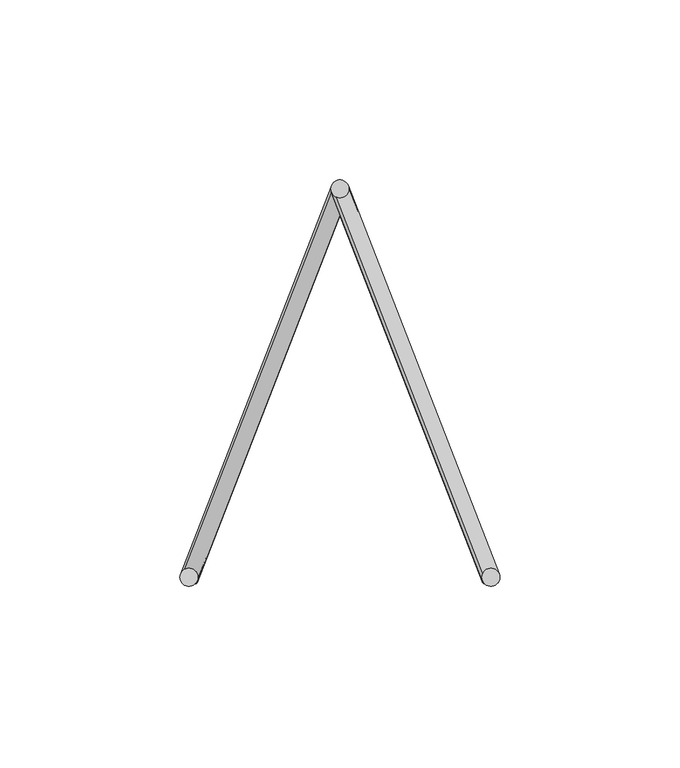
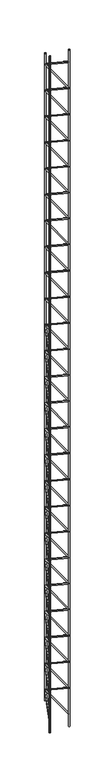
"""IFC4 building model written with IfcOpenShell, lengths in millimetres: proxy geometry, Pre-fab. (Vigota 2 - Pano 4)."""

from ifc_helpers import new_model, si_unit, point, frame, frame_2d, origin, origin_with_axes, origin_2d, place, context, project, spatial, circle_curve, trimmed, segment, composite_curve, outline, extrude, source, transform, mapped, element, save


def structural_framing_4307f6da(model_context):
    return source(origin(), model_context, "Body", "SweptSolid", [
        extrude(outline(composite_curve([segment(trimmed(circle_curve(origin_2d(), 2.5), [point((2.5, 0.0))], [point((-2.5, 0.0))], False, "CARTESIAN"), True, "CONTINUOUS"), segment(trimmed(circle_curve(origin_2d(), 2.5), [point((-2.5, 0.0))], [point((2.5, 0.0))], False, "CARTESIAN"), True, "CONTINUOUS")], self_intersect=False)), origin_with_axes(), (0.0, 0.0, 1.0), 3114.0),
        extrude(outline(composite_curve([segment(trimmed(circle_curve(frame_2d((-42.0, 108.0)), 2.5), [point((-39.5, 108.0))], [point((-44.5, 108.0))], False, "CARTESIAN"), True, "CONTINUOUS"), segment(trimmed(circle_curve(frame_2d((-42.0, 108.0)), 2.5), [point((-44.5, 108.0))], [point((-39.5, 108.0))], False, "CARTESIAN"), True, "CONTINUOUS")], self_intersect=False)), frame((0.0, 0.0, 67.0), z_axis=(0.0, 0.0, 1.0), x_axis=(1.0, 0.0, 0.0)), (0.0, 0.0, 1.0), 2980.0),
        extrude(outline(composite_curve([segment(trimmed(circle_curve(origin_2d(), 2.5), [point((2.5, 0.0))], [point((-2.5, 0.0))], False, "CARTESIAN"), True, "CONTINUOUS"), segment(trimmed(circle_curve(origin_2d(), 2.5), [point((-2.5, 0.0))], [point((2.5, 0.0))], False, "CARTESIAN"), True, "CONTINUOUS")], self_intersect=False)), frame((0.0, 0.0, 57.0), z_axis=(-0.3218603428886276, 0.8276408817707567, 0.4598004898837537), x_axis=(0.8192319205108605, -3.936835275445103e-11, 0.5734623443750141)), (0.0, 0.0, 1.0), 130.491379),
        extrude(outline(composite_curve([segment(trimmed(circle_curve(origin_2d(), 2.5), [point((2.5, 0.0))], [point((-2.5, 0.0))], False, "CARTESIAN"), True, "CONTINUOUS"), segment(trimmed(circle_curve(origin_2d(), 2.5), [point((-2.5, 0.0))], [point((2.5, 0.0))], False, "CARTESIAN"), True, "CONTINUOUS")], self_intersect=False)), frame((-42.0, 108.0, 117.0), z_axis=(0.3218603428886276, -0.8276408817707567, 0.4598004898837537), x_axis=(0.8192319205108605, -3.936835275445103e-11, -0.5734623443750141)), (0.0, 0.0, 1.0), 130.491379),
        extrude(outline(composite_curve([segment(trimmed(circle_curve(origin_2d(), 2.5), [point((2.5, 0.0))], [point((-2.5, 0.0))], False, "CARTESIAN"), True, "CONTINUOUS"), segment(trimmed(circle_curve(origin_2d(), 2.5), [point((-2.5, 0.0))], [point((2.5, 0.0))], False, "CARTESIAN"), True, "CONTINUOUS")], self_intersect=False)), frame((0.0, 0.0, 177.0), z_axis=(-0.3218603428886276, 0.8276408817707567, 0.4598004898837537), x_axis=(0.8192319205108605, -3.936835275445103e-11, 0.5734623443750141)), (0.0, 0.0, 1.0), 130.491379),
        extrude(outline(composite_curve([segment(trimmed(circle_curve(origin_2d(), 2.5), [point((2.5, 0.0))], [point((-2.5, 0.0))], False, "CARTESIAN"), True, "CONTINUOUS"), segment(trimmed(circle_curve(origin_2d(), 2.5), [point((-2.5, 0.0))], [point((2.5, 0.0))], False, "CARTESIAN"), True, "CONTINUOUS")], self_intersect=False)), frame((-42.0, 108.0, 237.0), z_axis=(0.3218603428886276, -0.8276408817707567, 0.4598004898837537), x_axis=(0.8192319205108605, -3.936835275445103e-11, -0.5734623443750141)), (0.0, 0.0, 1.0), 130.491379),
        extrude(outline(composite_curve([segment(trimmed(circle_curve(origin_2d(), 2.5), [point((2.5, 0.0))], [point((-2.5, 0.0))], False, "CARTESIAN"), True, "CONTINUOUS"), segment(trimmed(circle_curve(origin_2d(), 2.5), [point((-2.5, 0.0))], [point((2.5, 0.0))], False, "CARTESIAN"), True, "CONTINUOUS")], self_intersect=False)), frame((0.0, 0.0, 297.0), z_axis=(-0.3218603428886276, 0.8276408817707567, 0.4598004898837537), x_axis=(0.8192319205108605, -3.936835275445103e-11, 0.5734623443750141)), (0.0, 0.0, 1.0), 130.491379),
        extrude(outline(composite_curve([segment(trimmed(circle_curve(origin_2d(), 2.5), [point((2.5, 0.0))], [point((-2.5, 0.0))], False, "CARTESIAN"), True, "CONTINUOUS"), segment(trimmed(circle_curve(origin_2d(), 2.5), [point((-2.5, 0.0))], [point((2.5, 0.0))], False, "CARTESIAN"), True, "CONTINUOUS")], self_intersect=False)), frame((-42.0, 108.0, 357.0), z_axis=(0.3218603428886276, -0.8276408817707567, 0.4598004898837537), x_axis=(0.8192319205108605, -3.936835275445103e-11, -0.5734623443750141)), (0.0, 0.0, 1.0), 130.491379),
        extrude(outline(composite_curve([segment(trimmed(circle_curve(origin_2d(), 2.5), [point((2.5, 0.0))], [point((-2.5, 0.0))], False, "CARTESIAN"), True, "CONTINUOUS"), segment(trimmed(circle_curve(origin_2d(), 2.5), [point((-2.5, 0.0))], [point((2.5, 0.0))], False, "CARTESIAN"), True, "CONTINUOUS")], self_intersect=False)), frame((0.0, 0.0, 417.0), z_axis=(-0.3218603428886276, 0.8276408817707567, 0.4598004898837537), x_axis=(0.8192319205108605, -3.936835275445103e-11, 0.5734623443750141)), (0.0, 0.0, 1.0), 130.491379),
        extrude(outline(composite_curve([segment(trimmed(circle_curve(origin_2d(), 2.5), [point((2.5, 0.0))], [point((-2.5, 0.0))], False, "CARTESIAN"), True, "CONTINUOUS"), segment(trimmed(circle_curve(origin_2d(), 2.5), [point((-2.5, 0.0))], [point((2.5, 0.0))], False, "CARTESIAN"), True, "CONTINUOUS")], self_intersect=False)), frame((-42.0, 108.0, 477.0), z_axis=(0.3218603428886276, -0.8276408817707567, 0.4598004898837537), x_axis=(0.8192319205108605, -3.936835275445103e-11, -0.5734623443750141)), (0.0, 0.0, 1.0), 130.491379),
        extrude(outline(composite_curve([segment(trimmed(circle_curve(origin_2d(), 2.5), [point((2.5, 0.0))], [point((-2.5, 0.0))], False, "CARTESIAN"), True, "CONTINUOUS"), segment(trimmed(circle_curve(origin_2d(), 2.5), [point((-2.5, 0.0))], [point((2.5, 0.0))], False, "CARTESIAN"), True, "CONTINUOUS")], self_intersect=False)), frame((0.0, 0.0, 537.0), z_axis=(-0.3218603428886276, 0.8276408817707567, 0.4598004898837537), x_axis=(0.8192319205108605, -3.936835275445103e-11, 0.5734623443750141)), (0.0, 0.0, 1.0), 130.491379),
        extrude(outline(composite_curve([segment(trimmed(circle_curve(origin_2d(), 2.5), [point((2.5, 0.0))], [point((-2.5, 0.0))], False, "CARTESIAN"), True, "CONTINUOUS"), segment(trimmed(circle_curve(origin_2d(), 2.5), [point((-2.5, 0.0))], [point((2.5, 0.0))], False, "CARTESIAN"), True, "CONTINUOUS")], self_intersect=False)), frame((-42.0, 108.0, 597.0), z_axis=(0.3218603428886276, -0.8276408817707567, 0.4598004898837537), x_axis=(0.8192319205108605, -3.936835275445103e-11, -0.5734623443750141)), (0.0, 0.0, 1.0), 130.491379),
        extrude(outline(composite_curve([segment(trimmed(circle_curve(origin_2d(), 2.5), [point((2.5, 0.0))], [point((-2.5, 0.0))], False, "CARTESIAN"), True, "CONTINUOUS"), segment(trimmed(circle_curve(origin_2d(), 2.5), [point((-2.5, 0.0))], [point((2.5, 0.0))], False, "CARTESIAN"), True, "CONTINUOUS")], self_intersect=False)), frame((0.0, 0.0, 657.0), z_axis=(-0.3218603428886276, 0.8276408817707567, 0.4598004898837537), x_axis=(0.8192319205108605, -3.936835275445103e-11, 0.5734623443750141)), (0.0, 0.0, 1.0), 130.491379),
        extrude(outline(composite_curve([segment(trimmed(circle_curve(origin_2d(), 2.5), [point((2.5, 0.0))], [point((-2.5, 0.0))], False, "CARTESIAN"), True, "CONTINUOUS"), segment(trimmed(circle_curve(origin_2d(), 2.5), [point((-2.5, 0.0))], [point((2.5, 0.0))], False, "CARTESIAN"), True, "CONTINUOUS")], self_intersect=False)), frame((-42.0, 108.0, 717.0), z_axis=(0.3218603428886276, -0.8276408817707567, 0.4598004898837537), x_axis=(0.8192319205108605, -3.936835275445103e-11, -0.5734623443750141)), (0.0, 0.0, 1.0), 130.491379),
        extrude(outline(composite_curve([segment(trimmed(circle_curve(origin_2d(), 2.5), [point((2.5, 0.0))], [point((-2.5, 0.0))], False, "CARTESIAN"), True, "CONTINUOUS"), segment(trimmed(circle_curve(origin_2d(), 2.5), [point((-2.5, 0.0))], [point((2.5, 0.0))], False, "CARTESIAN"), True, "CONTINUOUS")], self_intersect=False)), frame((0.0, 0.0, 777.0), z_axis=(-0.3218603428886276, 0.8276408817707567, 0.4598004898837537), x_axis=(0.8192319205108605, -3.936835275445103e-11, 0.5734623443750141)), (0.0, 0.0, 1.0), 130.491379),
        extrude(outline(composite_curve([segment(trimmed(circle_curve(origin_2d(), 2.5), [point((2.5, 0.0))], [point((-2.5, 0.0))], False, "CARTESIAN"), True, "CONTINUOUS"), segment(trimmed(circle_curve(origin_2d(), 2.5), [point((-2.5, 0.0))], [point((2.5, 0.0))], False, "CARTESIAN"), True, "CONTINUOUS")], self_intersect=False)), frame((-42.0, 108.0, 837.0), z_axis=(0.3218603428886276, -0.8276408817707567, 0.4598004898837537), x_axis=(0.8192319205108605, -3.936835275445103e-11, -0.5734623443750141)), (0.0, 0.0, 1.0), 130.491379),
        extrude(outline(composite_curve([segment(trimmed(circle_curve(origin_2d(), 2.5), [point((2.5, 0.0))], [point((-2.5, 0.0))], False, "CARTESIAN"), True, "CONTINUOUS"), segment(trimmed(circle_curve(origin_2d(), 2.5), [point((-2.5, 0.0))], [point((2.5, 0.0))], False, "CARTESIAN"), True, "CONTINUOUS")], self_intersect=False)), frame((0.0, 0.0, 897.0), z_axis=(-0.3218603428886276, 0.8276408817707567, 0.4598004898837537), x_axis=(0.8192319205108605, -3.936835275445103e-11, 0.5734623443750141)), (0.0, 0.0, 1.0), 130.491379),
        extrude(outline(composite_curve([segment(trimmed(circle_curve(origin_2d(), 2.5), [point((2.5, 0.0))], [point((-2.5, 0.0))], False, "CARTESIAN"), True, "CONTINUOUS"), segment(trimmed(circle_curve(origin_2d(), 2.5), [point((-2.5, 0.0))], [point((2.5, 0.0))], False, "CARTESIAN"), True, "CONTINUOUS")], self_intersect=False)), frame((-42.0, 108.0, 957.0), z_axis=(0.3218603428886276, -0.8276408817707567, 0.4598004898837537), x_axis=(0.8192319205108605, -3.936835275445103e-11, -0.5734623443750141)), (0.0, 0.0, 1.0), 130.491379),
        extrude(outline(composite_curve([segment(trimmed(circle_curve(origin_2d(), 2.5), [point((2.5, 0.0))], [point((-2.5, 0.0))], False, "CARTESIAN"), True, "CONTINUOUS"), segment(trimmed(circle_curve(origin_2d(), 2.5), [point((-2.5, 0.0))], [point((2.5, 0.0))], False, "CARTESIAN"), True, "CONTINUOUS")], self_intersect=False)), frame((0.0, 0.0, 1017.0), z_axis=(-0.3218603428886276, 0.8276408817707567, 0.4598004898837537), x_axis=(0.8192319205108605, -3.936835275445103e-11, 0.5734623443750141)), (0.0, 0.0, 1.0), 130.491379),
        extrude(outline(composite_curve([segment(trimmed(circle_curve(origin_2d(), 2.5), [point((2.5, 0.0))], [point((-2.5, 0.0))], False, "CARTESIAN"), True, "CONTINUOUS"), segment(trimmed(circle_curve(origin_2d(), 2.5), [point((-2.5, 0.0))], [point((2.5, 0.0))], False, "CARTESIAN"), True, "CONTINUOUS")], self_intersect=False)), frame((-42.0, 108.0, 1077.0), z_axis=(0.3218603428886276, -0.8276408817707567, 0.4598004898837537), x_axis=(0.8192319205108605, -3.936835275445103e-11, -0.5734623443750141)), (0.0, 0.0, 1.0), 130.491379),
        extrude(outline(composite_curve([segment(trimmed(circle_curve(origin_2d(), 2.5), [point((2.5, 0.0))], [point((-2.5, 0.0))], False, "CARTESIAN"), True, "CONTINUOUS"), segment(trimmed(circle_curve(origin_2d(), 2.5), [point((-2.5, 0.0))], [point((2.5, 0.0))], False, "CARTESIAN"), True, "CONTINUOUS")], self_intersect=False)), frame((0.0, 0.0, 1137.0), z_axis=(-0.3218603428886276, 0.8276408817707567, 0.4598004898837537), x_axis=(0.8192319205108605, -3.936835275445103e-11, 0.5734623443750141)), (0.0, 0.0, 1.0), 130.491379),
        extrude(outline(composite_curve([segment(trimmed(circle_curve(origin_2d(), 2.5), [point((2.5, 0.0))], [point((-2.5, 0.0))], False, "CARTESIAN"), True, "CONTINUOUS"), segment(trimmed(circle_curve(origin_2d(), 2.5), [point((-2.5, 0.0))], [point((2.5, 0.0))], False, "CARTESIAN"), True, "CONTINUOUS")], self_intersect=False)), frame((-42.0, 108.0, 1197.0), z_axis=(0.3218603428886276, -0.8276408817707567, 0.4598004898837537), x_axis=(0.8192319205108605, -3.936835275445103e-11, -0.5734623443750141)), (0.0, 0.0, 1.0), 130.491379),
        extrude(outline(composite_curve([segment(trimmed(circle_curve(origin_2d(), 2.5), [point((2.5, 0.0))], [point((-2.5, 0.0))], False, "CARTESIAN"), True, "CONTINUOUS"), segment(trimmed(circle_curve(origin_2d(), 2.5), [point((-2.5, 0.0))], [point((2.5, 0.0))], False, "CARTESIAN"), True, "CONTINUOUS")], self_intersect=False)), frame((0.0, 0.0, 1257.0), z_axis=(-0.3218603428886276, 0.8276408817707567, 0.4598004898837537), x_axis=(0.8192319205108605, -3.936835275445103e-11, 0.5734623443750141)), (0.0, 0.0, 1.0), 130.491379),
        extrude(outline(composite_curve([segment(trimmed(circle_curve(origin_2d(), 2.5), [point((2.5, 0.0))], [point((-2.5, 0.0))], False, "CARTESIAN"), True, "CONTINUOUS"), segment(trimmed(circle_curve(origin_2d(), 2.5), [point((-2.5, 0.0))], [point((2.5, 0.0))], False, "CARTESIAN"), True, "CONTINUOUS")], self_intersect=False)), frame((-42.0, 108.0, 1317.0), z_axis=(0.3218603428886276, -0.8276408817707567, 0.4598004898837537), x_axis=(0.8192319205108605, -3.936835275445103e-11, -0.5734623443750141)), (0.0, 0.0, 1.0), 130.491379),
        extrude(outline(composite_curve([segment(trimmed(circle_curve(origin_2d(), 2.5), [point((2.5, 0.0))], [point((-2.5, 0.0))], False, "CARTESIAN"), True, "CONTINUOUS"), segment(trimmed(circle_curve(origin_2d(), 2.5), [point((-2.5, 0.0))], [point((2.5, 0.0))], False, "CARTESIAN"), True, "CONTINUOUS")], self_intersect=False)), frame((0.0, 0.0, 1377.0), z_axis=(-0.3218603428886276, 0.8276408817707567, 0.4598004898837537), x_axis=(0.8192319205108605, -3.936835275445103e-11, 0.5734623443750141)), (0.0, 0.0, 1.0), 130.491379),
        extrude(outline(composite_curve([segment(trimmed(circle_curve(origin_2d(), 2.5), [point((2.5, 0.0))], [point((-2.5, 0.0))], False, "CARTESIAN"), True, "CONTINUOUS"), segment(trimmed(circle_curve(origin_2d(), 2.5), [point((-2.5, 0.0))], [point((2.5, 0.0))], False, "CARTESIAN"), True, "CONTINUOUS")], self_intersect=False)), frame((-42.0, 108.0, 1437.0), z_axis=(0.3218603428886276, -0.8276408817707567, 0.4598004898837537), x_axis=(0.8192319205108605, -3.936835275445103e-11, -0.5734623443750141)), (0.0, 0.0, 1.0), 130.491379),
        extrude(outline(composite_curve([segment(trimmed(circle_curve(origin_2d(), 2.5), [point((2.5, 0.0))], [point((-2.5, 0.0))], False, "CARTESIAN"), True, "CONTINUOUS"), segment(trimmed(circle_curve(origin_2d(), 2.5), [point((-2.5, 0.0))], [point((2.5, 0.0))], False, "CARTESIAN"), True, "CONTINUOUS")], self_intersect=False)), frame((0.0, 0.0, 1497.0), z_axis=(-0.3218603428886276, 0.8276408817707567, 0.4598004898837537), x_axis=(0.8192319205108605, -3.936835275445103e-11, 0.5734623443750141)), (0.0, 0.0, 1.0), 130.491379),
        extrude(outline(composite_curve([segment(trimmed(circle_curve(origin_2d(), 2.5), [point((2.5, 0.0))], [point((-2.5, 0.0))], False, "CARTESIAN"), True, "CONTINUOUS"), segment(trimmed(circle_curve(origin_2d(), 2.5), [point((-2.5, 0.0))], [point((2.5, 0.0))], False, "CARTESIAN"), True, "CONTINUOUS")], self_intersect=False)), frame((-42.0, 108.0, 1557.0), z_axis=(0.3218603428886276, -0.8276408817707567, 0.4598004898837537), x_axis=(0.8192319205108605, -3.936835275445103e-11, -0.5734623443750141)), (0.0, 0.0, 1.0), 130.491379),
        extrude(outline(composite_curve([segment(trimmed(circle_curve(origin_2d(), 2.5), [point((2.5, 0.0))], [point((-2.5, 0.0))], False, "CARTESIAN"), True, "CONTINUOUS"), segment(trimmed(circle_curve(origin_2d(), 2.5), [point((-2.5, 0.0))], [point((2.5, 0.0))], False, "CARTESIAN"), True, "CONTINUOUS")], self_intersect=False)), frame((0.0, 0.0, 1617.0), z_axis=(-0.3218603428886276, 0.8276408817707567, 0.4598004898837537), x_axis=(0.8192319205108605, -3.936835275445103e-11, 0.5734623443750141)), (0.0, 0.0, 1.0), 130.491379),
        extrude(outline(composite_curve([segment(trimmed(circle_curve(origin_2d(), 2.5), [point((2.5, 0.0))], [point((-2.5, 0.0))], False, "CARTESIAN"), True, "CONTINUOUS"), segment(trimmed(circle_curve(origin_2d(), 2.5), [point((-2.5, 0.0))], [point((2.5, 0.0))], False, "CARTESIAN"), True, "CONTINUOUS")], self_intersect=False)), frame((-42.0, 108.0, 1677.0), z_axis=(0.3218603428886276, -0.8276408817707567, 0.4598004898837537), x_axis=(0.8192319205108605, -3.936835275445103e-11, -0.5734623443750141)), (0.0, 0.0, 1.0), 130.491379),
        extrude(outline(composite_curve([segment(trimmed(circle_curve(origin_2d(), 2.5), [point((2.5, 0.0))], [point((-2.5, 0.0))], False, "CARTESIAN"), True, "CONTINUOUS"), segment(trimmed(circle_curve(origin_2d(), 2.5), [point((-2.5, 0.0))], [point((2.5, 0.0))], False, "CARTESIAN"), True, "CONTINUOUS")], self_intersect=False)), frame((0.0, 0.0, 1737.0), z_axis=(-0.3218603428886276, 0.8276408817707567, 0.4598004898837537), x_axis=(0.8192319205108605, -3.936835275445103e-11, 0.5734623443750141)), (0.0, 0.0, 1.0), 130.491379),
        extrude(outline(composite_curve([segment(trimmed(circle_curve(origin_2d(), 2.5), [point((2.5, 0.0))], [point((-2.5, 0.0))], False, "CARTESIAN"), True, "CONTINUOUS"), segment(trimmed(circle_curve(origin_2d(), 2.5), [point((-2.5, 0.0))], [point((2.5, 0.0))], False, "CARTESIAN"), True, "CONTINUOUS")], self_intersect=False)), frame((-42.0, 108.0, 1797.0), z_axis=(0.3218603428886276, -0.8276408817707567, 0.4598004898837537), x_axis=(0.8192319205108605, -3.936835275445103e-11, -0.5734623443750141)), (0.0, 0.0, 1.0), 130.491379),
        extrude(outline(composite_curve([segment(trimmed(circle_curve(origin_2d(), 2.5), [point((2.5, 0.0))], [point((-2.5, 0.0))], False, "CARTESIAN"), True, "CONTINUOUS"), segment(trimmed(circle_curve(origin_2d(), 2.5), [point((-2.5, 0.0))], [point((2.5, 0.0))], False, "CARTESIAN"), True, "CONTINUOUS")], self_intersect=False)), frame((0.0, 0.0, 1857.0), z_axis=(-0.3218603428886276, 0.8276408817707567, 0.4598004898837537), x_axis=(0.8192319205108605, -3.936835275445103e-11, 0.5734623443750141)), (0.0, 0.0, 1.0), 130.491379),
        extrude(outline(composite_curve([segment(trimmed(circle_curve(origin_2d(), 2.5), [point((2.5, 0.0))], [point((-2.5, 0.0))], False, "CARTESIAN"), True, "CONTINUOUS"), segment(trimmed(circle_curve(origin_2d(), 2.5), [point((-2.5, 0.0))], [point((2.5, 0.0))], False, "CARTESIAN"), True, "CONTINUOUS")], self_intersect=False)), frame((-42.0, 108.0, 1917.0), z_axis=(0.3218603428886276, -0.8276408817707567, 0.4598004898837537), x_axis=(0.8192319205108605, -3.936835275445103e-11, -0.5734623443750141)), (0.0, 0.0, 1.0), 130.491379),
        extrude(outline(composite_curve([segment(trimmed(circle_curve(origin_2d(), 2.5), [point((2.5, 0.0))], [point((-2.5, 0.0))], False, "CARTESIAN"), True, "CONTINUOUS"), segment(trimmed(circle_curve(origin_2d(), 2.5), [point((-2.5, 0.0))], [point((2.5, 0.0))], False, "CARTESIAN"), True, "CONTINUOUS")], self_intersect=False)), frame((0.0, 0.0, 1977.0), z_axis=(-0.3218603428886276, 0.8276408817707567, 0.4598004898837537), x_axis=(0.8192319205108605, -3.936835275445103e-11, 0.5734623443750141)), (0.0, 0.0, 1.0), 130.491379),
        extrude(outline(composite_curve([segment(trimmed(circle_curve(origin_2d(), 2.5), [point((2.5, 0.0))], [point((-2.5, 0.0))], False, "CARTESIAN"), True, "CONTINUOUS"), segment(trimmed(circle_curve(origin_2d(), 2.5), [point((-2.5, 0.0))], [point((2.5, 0.0))], False, "CARTESIAN"), True, "CONTINUOUS")], self_intersect=False)), frame((-42.0, 108.0, 2037.0), z_axis=(0.3218603428886276, -0.8276408817707567, 0.4598004898837537), x_axis=(0.8192319205108605, -3.936835275445103e-11, -0.5734623443750141)), (0.0, 0.0, 1.0), 130.491379),
        extrude(outline(composite_curve([segment(trimmed(circle_curve(origin_2d(), 2.5), [point((2.5, 0.0))], [point((-2.5, 0.0))], False, "CARTESIAN"), True, "CONTINUOUS"), segment(trimmed(circle_curve(origin_2d(), 2.5), [point((-2.5, 0.0))], [point((2.5, 0.0))], False, "CARTESIAN"), True, "CONTINUOUS")], self_intersect=False)), frame((0.0, 0.0, 2097.0), z_axis=(-0.3218603428886276, 0.8276408817707567, 0.4598004898837537), x_axis=(0.8192319205108605, -3.936835275445103e-11, 0.5734623443750141)), (0.0, 0.0, 1.0), 130.491379),
        extrude(outline(composite_curve([segment(trimmed(circle_curve(origin_2d(), 2.5), [point((2.5, 0.0))], [point((-2.5, 0.0))], False, "CARTESIAN"), True, "CONTINUOUS"), segment(trimmed(circle_curve(origin_2d(), 2.5), [point((-2.5, 0.0))], [point((2.5, 0.0))], False, "CARTESIAN"), True, "CONTINUOUS")], self_intersect=False)), frame((-42.0, 108.0, 2157.0), z_axis=(0.3218603428886276, -0.8276408817707567, 0.4598004898837537), x_axis=(0.8192319205108605, -3.936835275445103e-11, -0.5734623443750141)), (0.0, 0.0, 1.0), 130.491379),
        extrude(outline(composite_curve([segment(trimmed(circle_curve(origin_2d(), 2.5), [point((2.5, 0.0))], [point((-2.5, 0.0))], False, "CARTESIAN"), True, "CONTINUOUS"), segment(trimmed(circle_curve(origin_2d(), 2.5), [point((-2.5, 0.0))], [point((2.5, 0.0))], False, "CARTESIAN"), True, "CONTINUOUS")], self_intersect=False)), frame((0.0, 0.0, 2217.0), z_axis=(-0.3218603428886276, 0.8276408817707567, 0.4598004898837537), x_axis=(0.8192319205108605, -3.936835275445103e-11, 0.5734623443750141)), (0.0, 0.0, 1.0), 130.491379),
        extrude(outline(composite_curve([segment(trimmed(circle_curve(origin_2d(), 2.5), [point((2.5, 0.0))], [point((-2.5, 0.0))], False, "CARTESIAN"), True, "CONTINUOUS"), segment(trimmed(circle_curve(origin_2d(), 2.5), [point((-2.5, 0.0))], [point((2.5, 0.0))], False, "CARTESIAN"), True, "CONTINUOUS")], self_intersect=False)), frame((-42.0, 108.0, 2277.0), z_axis=(0.3218603428886276, -0.8276408817707567, 0.4598004898837537), x_axis=(0.8192319205108605, -3.936835275445103e-11, -0.5734623443750141)), (0.0, 0.0, 1.0), 130.491379),
        extrude(outline(composite_curve([segment(trimmed(circle_curve(origin_2d(), 2.5), [point((2.5, 0.0))], [point((-2.5, 0.0))], False, "CARTESIAN"), True, "CONTINUOUS"), segment(trimmed(circle_curve(origin_2d(), 2.5), [point((-2.5, 0.0))], [point((2.5, 0.0))], False, "CARTESIAN"), True, "CONTINUOUS")], self_intersect=False)), frame((0.0, 0.0, 2337.0), z_axis=(-0.3218603428886276, 0.8276408817707567, 0.4598004898837537), x_axis=(0.8192319205108605, -3.936835275445103e-11, 0.5734623443750141)), (0.0, 0.0, 1.0), 130.491379),
        extrude(outline(composite_curve([segment(trimmed(circle_curve(origin_2d(), 2.5), [point((2.5, 0.0))], [point((-2.5, 0.0))], False, "CARTESIAN"), True, "CONTINUOUS"), segment(trimmed(circle_curve(origin_2d(), 2.5), [point((-2.5, 0.0))], [point((2.5, 0.0))], False, "CARTESIAN"), True, "CONTINUOUS")], self_intersect=False)), frame((-42.0, 108.0, 2397.0), z_axis=(0.3218603428886276, -0.8276408817707567, 0.4598004898837537), x_axis=(0.8192319205108605, -3.936835275445103e-11, -0.5734623443750141)), (0.0, 0.0, 1.0), 130.491379),
        extrude(outline(composite_curve([segment(trimmed(circle_curve(origin_2d(), 2.5), [point((2.5, 0.0))], [point((-2.5, 0.0))], False, "CARTESIAN"), True, "CONTINUOUS"), segment(trimmed(circle_curve(origin_2d(), 2.5), [point((-2.5, 0.0))], [point((2.5, 0.0))], False, "CARTESIAN"), True, "CONTINUOUS")], self_intersect=False)), frame((0.0, 0.0, 2457.0), z_axis=(-0.3218603428886276, 0.8276408817707567, 0.4598004898837537), x_axis=(0.8192319205108605, -3.936835275445103e-11, 0.5734623443750141)), (0.0, 0.0, 1.0), 130.491379),
        extrude(outline(composite_curve([segment(trimmed(circle_curve(origin_2d(), 2.5), [point((2.5, 0.0))], [point((-2.5, 0.0))], False, "CARTESIAN"), True, "CONTINUOUS"), segment(trimmed(circle_curve(origin_2d(), 2.5), [point((-2.5, 0.0))], [point((2.5, 0.0))], False, "CARTESIAN"), True, "CONTINUOUS")], self_intersect=False)), frame((-42.0, 108.0, 2517.0), z_axis=(0.3218603428886276, -0.8276408817707567, 0.4598004898837537), x_axis=(0.8192319205108605, -3.936835275445103e-11, -0.5734623443750141)), (0.0, 0.0, 1.0), 130.491379),
        extrude(outline(composite_curve([segment(trimmed(circle_curve(origin_2d(), 2.5), [point((2.5, 0.0))], [point((-2.5, 0.0))], False, "CARTESIAN"), True, "CONTINUOUS"), segment(trimmed(circle_curve(origin_2d(), 2.5), [point((-2.5, 0.0))], [point((2.5, 0.0))], False, "CARTESIAN"), True, "CONTINUOUS")], self_intersect=False)), frame((0.0, 0.0, 2577.0), z_axis=(-0.3218603428886276, 0.8276408817707567, 0.4598004898837537), x_axis=(0.8192319205108605, -3.936835275445103e-11, 0.5734623443750141)), (0.0, 0.0, 1.0), 130.491379),
        extrude(outline(composite_curve([segment(trimmed(circle_curve(origin_2d(), 2.5), [point((2.5, 0.0))], [point((-2.5, 0.0))], False, "CARTESIAN"), True, "CONTINUOUS"), segment(trimmed(circle_curve(origin_2d(), 2.5), [point((-2.5, 0.0))], [point((2.5, 0.0))], False, "CARTESIAN"), True, "CONTINUOUS")], self_intersect=False)), frame((-42.0, 108.0, 2637.0), z_axis=(0.3218603428886276, -0.8276408817707567, 0.4598004898837537), x_axis=(0.8192319205108605, -3.936835275445103e-11, -0.5734623443750141)), (0.0, 0.0, 1.0), 130.491379),
        extrude(outline(composite_curve([segment(trimmed(circle_curve(origin_2d(), 2.5), [point((2.5, 0.0))], [point((-2.5, 0.0))], False, "CARTESIAN"), True, "CONTINUOUS"), segment(trimmed(circle_curve(origin_2d(), 2.5), [point((-2.5, 0.0))], [point((2.5, 0.0))], False, "CARTESIAN"), True, "CONTINUOUS")], self_intersect=False)), frame((0.0, 0.0, 2697.0), z_axis=(-0.3218603428886276, 0.8276408817707567, 0.4598004898837537), x_axis=(0.8192319205108605, -3.936835275445103e-11, 0.5734623443750141)), (0.0, 0.0, 1.0), 130.491379),
        extrude(outline(composite_curve([segment(trimmed(circle_curve(origin_2d(), 2.5), [point((2.5, 0.0))], [point((-2.5, 0.0))], False, "CARTESIAN"), True, "CONTINUOUS"), segment(trimmed(circle_curve(origin_2d(), 2.5), [point((-2.5, 0.0))], [point((2.5, 0.0))], False, "CARTESIAN"), True, "CONTINUOUS")], self_intersect=False)), frame((-42.0, 108.0, 2757.0), z_axis=(0.3218603428886276, -0.8276408817707567, 0.4598004898837537), x_axis=(0.8192319205108605, -3.936835275445103e-11, -0.5734623443750141)), (0.0, 0.0, 1.0), 130.491379),
        extrude(outline(composite_curve([segment(trimmed(circle_curve(origin_2d(), 2.5), [point((2.5, 0.0))], [point((-2.5, 0.0))], False, "CARTESIAN"), True, "CONTINUOUS"), segment(trimmed(circle_curve(origin_2d(), 2.5), [point((-2.5, 0.0))], [point((2.5, 0.0))], False, "CARTESIAN"), True, "CONTINUOUS")], self_intersect=False)), frame((0.0, 0.0, 2817.0), z_axis=(-0.3218603428886276, 0.8276408817707567, 0.4598004898837537), x_axis=(0.8192319205108605, -3.936835275445103e-11, 0.5734623443750141)), (0.0, 0.0, 1.0), 130.491379),
        extrude(outline(composite_curve([segment(trimmed(circle_curve(origin_2d(), 2.5), [point((2.5, 0.0))], [point((-2.5, 0.0))], False, "CARTESIAN"), True, "CONTINUOUS"), segment(trimmed(circle_curve(origin_2d(), 2.5), [point((-2.5, 0.0))], [point((2.5, 0.0))], False, "CARTESIAN"), True, "CONTINUOUS")], self_intersect=False)), frame((-42.0, 108.0, 2877.0), z_axis=(0.3218603428886276, -0.8276408817707567, 0.4598004898837537), x_axis=(0.8192319205108605, -3.936835275445103e-11, -0.5734623443750141)), (0.0, 0.0, 1.0), 130.491379),
        extrude(outline(composite_curve([segment(trimmed(circle_curve(origin_2d(), 2.5), [point((2.5, 0.0))], [point((-2.5, 0.0))], False, "CARTESIAN"), True, "CONTINUOUS"), segment(trimmed(circle_curve(origin_2d(), 2.5), [point((-2.5, 0.0))], [point((2.5, 0.0))], False, "CARTESIAN"), True, "CONTINUOUS")], self_intersect=False)), frame((0.0, 0.0, 2937.0), z_axis=(-0.3218603428886276, 0.8276408817707567, 0.4598004898837537), x_axis=(0.8192319205108605, -3.936835275445103e-11, 0.5734623443750141)), (0.0, 0.0, 1.0), 130.491379),
        extrude(outline(composite_curve([segment(trimmed(circle_curve(origin_2d(), 2.5), [point((2.5, 0.0))], [point((-2.5, 0.0))], False, "CARTESIAN"), True, "CONTINUOUS"), segment(trimmed(circle_curve(origin_2d(), 2.5), [point((-2.5, 0.0))], [point((2.5, 0.0))], False, "CARTESIAN"), True, "CONTINUOUS")], self_intersect=False)), frame((-42.0, 108.0, 2997.0), z_axis=(0.3218603428886276, -0.8276408817707567, 0.4598004898837537), x_axis=(0.8192319205108605, -3.936835275445103e-11, -0.5734623443750141)), (0.0, 0.0, 1.0), 130.491379),
        extrude(outline(composite_curve([segment(trimmed(circle_curve(frame_2d((-84.0, 0.0)), 2.5), [point((-81.5, 0.0))], [point((-86.5, 0.0))], False, "CARTESIAN"), True, "CONTINUOUS"), segment(trimmed(circle_curve(frame_2d((-84.0, 0.0)), 2.5), [point((-86.5, 0.0))], [point((-81.5, 0.0))], False, "CARTESIAN"), True, "CONTINUOUS")], self_intersect=False)), origin_with_axes(), (0.0, 0.0, 1.0), 3114.0),
        extrude(outline(composite_curve([segment(trimmed(circle_curve(origin_2d(), 2.5), [point((2.5, 0.0))], [point((-2.5, 0.0))], False, "CARTESIAN"), True, "CONTINUOUS"), segment(trimmed(circle_curve(origin_2d(), 2.5), [point((-2.5, 0.0))], [point((2.5, 0.0))], False, "CARTESIAN"), True, "CONTINUOUS")], self_intersect=False)), frame((-84.0, 0.0, 57.0), z_axis=(0.3218603428886276, 0.8276408817707567, 0.4598004898837537), x_axis=(0.8192319205108605, 3.936835275445103e-11, -0.5734623443750141)), (0.0, 0.0, 1.0), 130.491379),
        extrude(outline(composite_curve([segment(trimmed(circle_curve(origin_2d(), 2.5), [point((2.5, 0.0))], [point((-2.5, 0.0))], False, "CARTESIAN"), True, "CONTINUOUS"), segment(trimmed(circle_curve(origin_2d(), 2.5), [point((-2.5, 0.0))], [point((2.5, 0.0))], False, "CARTESIAN"), True, "CONTINUOUS")], self_intersect=False)), frame((-42.0, 108.0, 117.0), z_axis=(-0.3218603428886276, -0.8276408817707567, 0.4598004898837537), x_axis=(0.8192319205108605, 3.936835275445103e-11, 0.5734623443750141)), (0.0, 0.0, 1.0), 130.491379),
        extrude(outline(composite_curve([segment(trimmed(circle_curve(origin_2d(), 2.5), [point((2.5, 0.0))], [point((-2.5, 0.0))], False, "CARTESIAN"), True, "CONTINUOUS"), segment(trimmed(circle_curve(origin_2d(), 2.5), [point((-2.5, 0.0))], [point((2.5, 0.0))], False, "CARTESIAN"), True, "CONTINUOUS")], self_intersect=False)), frame((-84.0, 0.0, 177.0), z_axis=(0.3218603428886276, 0.8276408817707567, 0.4598004898837537), x_axis=(0.8192319205108605, 3.936835275445103e-11, -0.5734623443750141)), (0.0, 0.0, 1.0), 130.491379),
        extrude(outline(composite_curve([segment(trimmed(circle_curve(origin_2d(), 2.5), [point((2.5, 0.0))], [point((-2.5, 0.0))], False, "CARTESIAN"), True, "CONTINUOUS"), segment(trimmed(circle_curve(origin_2d(), 2.5), [point((-2.5, 0.0))], [point((2.5, 0.0))], False, "CARTESIAN"), True, "CONTINUOUS")], self_intersect=False)), frame((-42.0, 108.0, 237.0), z_axis=(-0.3218603428886276, -0.8276408817707567, 0.4598004898837537), x_axis=(0.8192319205108605, 3.936835275445103e-11, 0.5734623443750141)), (0.0, 0.0, 1.0), 130.491379),
        extrude(outline(composite_curve([segment(trimmed(circle_curve(origin_2d(), 2.5), [point((2.5, 0.0))], [point((-2.5, 0.0))], False, "CARTESIAN"), True, "CONTINUOUS"), segment(trimmed(circle_curve(origin_2d(), 2.5), [point((-2.5, 0.0))], [point((2.5, 0.0))], False, "CARTESIAN"), True, "CONTINUOUS")], self_intersect=False)), frame((-84.0, 0.0, 297.0), z_axis=(0.3218603428886276, 0.8276408817707567, 0.4598004898837537), x_axis=(0.8192319205108605, 3.936835275445103e-11, -0.5734623443750141)), (0.0, 0.0, 1.0), 130.491379),
        extrude(outline(composite_curve([segment(trimmed(circle_curve(origin_2d(), 2.5), [point((2.5, 0.0))], [point((-2.5, 0.0))], False, "CARTESIAN"), True, "CONTINUOUS"), segment(trimmed(circle_curve(origin_2d(), 2.5), [point((-2.5, 0.0))], [point((2.5, 0.0))], False, "CARTESIAN"), True, "CONTINUOUS")], self_intersect=False)), frame((-42.0, 108.0, 357.0), z_axis=(-0.3218603428886276, -0.8276408817707567, 0.4598004898837537), x_axis=(0.8192319205108605, 3.936835275445103e-11, 0.5734623443750141)), (0.0, 0.0, 1.0), 130.491379),
        extrude(outline(composite_curve([segment(trimmed(circle_curve(origin_2d(), 2.5), [point((2.5, 0.0))], [point((-2.5, 0.0))], False, "CARTESIAN"), True, "CONTINUOUS"), segment(trimmed(circle_curve(origin_2d(), 2.5), [point((-2.5, 0.0))], [point((2.5, 0.0))], False, "CARTESIAN"), True, "CONTINUOUS")], self_intersect=False)), frame((-84.0, 0.0, 417.0), z_axis=(0.3218603428886276, 0.8276408817707567, 0.4598004898837537), x_axis=(0.8192319205108605, 3.936835275445103e-11, -0.5734623443750141)), (0.0, 0.0, 1.0), 130.491379),
        extrude(outline(composite_curve([segment(trimmed(circle_curve(origin_2d(), 2.5), [point((2.5, 0.0))], [point((-2.5, 0.0))], False, "CARTESIAN"), True, "CONTINUOUS"), segment(trimmed(circle_curve(origin_2d(), 2.5), [point((-2.5, 0.0))], [point((2.5, 0.0))], False, "CARTESIAN"), True, "CONTINUOUS")], self_intersect=False)), frame((-42.0, 108.0, 477.0), z_axis=(-0.3218603428886276, -0.8276408817707567, 0.4598004898837537), x_axis=(0.8192319205108605, 3.936835275445103e-11, 0.5734623443750141)), (0.0, 0.0, 1.0), 130.491379),
        extrude(outline(composite_curve([segment(trimmed(circle_curve(origin_2d(), 2.5), [point((2.5, 0.0))], [point((-2.5, 0.0))], False, "CARTESIAN"), True, "CONTINUOUS"), segment(trimmed(circle_curve(origin_2d(), 2.5), [point((-2.5, 0.0))], [point((2.5, 0.0))], False, "CARTESIAN"), True, "CONTINUOUS")], self_intersect=False)), frame((-84.0, 0.0, 537.0), z_axis=(0.3218603428886276, 0.8276408817707567, 0.4598004898837537), x_axis=(0.8192319205108605, 3.936835275445103e-11, -0.5734623443750141)), (0.0, 0.0, 1.0), 130.491379),
        extrude(outline(composite_curve([segment(trimmed(circle_curve(origin_2d(), 2.5), [point((2.5, 0.0))], [point((-2.5, 0.0))], False, "CARTESIAN"), True, "CONTINUOUS"), segment(trimmed(circle_curve(origin_2d(), 2.5), [point((-2.5, 0.0))], [point((2.5, 0.0))], False, "CARTESIAN"), True, "CONTINUOUS")], self_intersect=False)), frame((-42.0, 108.0, 597.0), z_axis=(-0.3218603428886276, -0.8276408817707567, 0.4598004898837537), x_axis=(0.8192319205108605, 3.936835275445103e-11, 0.5734623443750141)), (0.0, 0.0, 1.0), 130.491379),
        extrude(outline(composite_curve([segment(trimmed(circle_curve(origin_2d(), 2.5), [point((2.5, 0.0))], [point((-2.5, 0.0))], False, "CARTESIAN"), True, "CONTINUOUS"), segment(trimmed(circle_curve(origin_2d(), 2.5), [point((-2.5, 0.0))], [point((2.5, 0.0))], False, "CARTESIAN"), True, "CONTINUOUS")], self_intersect=False)), frame((-84.0, 0.0, 657.0), z_axis=(0.3218603428886276, 0.8276408817707567, 0.4598004898837537), x_axis=(0.8192319205108605, 3.936835275445103e-11, -0.5734623443750141)), (0.0, 0.0, 1.0), 130.491379),
        extrude(outline(composite_curve([segment(trimmed(circle_curve(origin_2d(), 2.5), [point((2.5, 0.0))], [point((-2.5, 0.0))], False, "CARTESIAN"), True, "CONTINUOUS"), segment(trimmed(circle_curve(origin_2d(), 2.5), [point((-2.5, 0.0))], [point((2.5, 0.0))], False, "CARTESIAN"), True, "CONTINUOUS")], self_intersect=False)), frame((-42.0, 108.0, 717.0), z_axis=(-0.3218603428886276, -0.8276408817707567, 0.4598004898837537), x_axis=(0.8192319205108605, 3.936835275445103e-11, 0.5734623443750141)), (0.0, 0.0, 1.0), 130.491379),
        extrude(outline(composite_curve([segment(trimmed(circle_curve(origin_2d(), 2.5), [point((2.5, 0.0))], [point((-2.5, 0.0))], False, "CARTESIAN"), True, "CONTINUOUS"), segment(trimmed(circle_curve(origin_2d(), 2.5), [point((-2.5, 0.0))], [point((2.5, 0.0))], False, "CARTESIAN"), True, "CONTINUOUS")], self_intersect=False)), frame((-84.0, 0.0, 777.0), z_axis=(0.3218603428886276, 0.8276408817707567, 0.4598004898837537), x_axis=(0.8192319205108605, 3.936835275445103e-11, -0.5734623443750141)), (0.0, 0.0, 1.0), 130.491379),
        extrude(outline(composite_curve([segment(trimmed(circle_curve(origin_2d(), 2.5), [point((2.5, 0.0))], [point((-2.5, 0.0))], False, "CARTESIAN"), True, "CONTINUOUS"), segment(trimmed(circle_curve(origin_2d(), 2.5), [point((-2.5, 0.0))], [point((2.5, 0.0))], False, "CARTESIAN"), True, "CONTINUOUS")], self_intersect=False)), frame((-42.0, 108.0, 837.0), z_axis=(-0.3218603428886276, -0.8276408817707567, 0.4598004898837537), x_axis=(0.8192319205108605, 3.936835275445103e-11, 0.5734623443750141)), (0.0, 0.0, 1.0), 130.491379),
        extrude(outline(composite_curve([segment(trimmed(circle_curve(origin_2d(), 2.5), [point((2.5, 0.0))], [point((-2.5, 0.0))], False, "CARTESIAN"), True, "CONTINUOUS"), segment(trimmed(circle_curve(origin_2d(), 2.5), [point((-2.5, 0.0))], [point((2.5, 0.0))], False, "CARTESIAN"), True, "CONTINUOUS")], self_intersect=False)), frame((-84.0, 0.0, 897.0), z_axis=(0.3218603428886276, 0.8276408817707567, 0.4598004898837537), x_axis=(0.8192319205108605, 3.936835275445103e-11, -0.5734623443750141)), (0.0, 0.0, 1.0), 130.491379),
        extrude(outline(composite_curve([segment(trimmed(circle_curve(origin_2d(), 2.5), [point((2.5, 0.0))], [point((-2.5, 0.0))], False, "CARTESIAN"), True, "CONTINUOUS"), segment(trimmed(circle_curve(origin_2d(), 2.5), [point((-2.5, 0.0))], [point((2.5, 0.0))], False, "CARTESIAN"), True, "CONTINUOUS")], self_intersect=False)), frame((-42.0, 108.0, 957.0), z_axis=(-0.3218603428886276, -0.8276408817707567, 0.4598004898837537), x_axis=(0.8192319205108605, 3.936835275445103e-11, 0.5734623443750141)), (0.0, 0.0, 1.0), 130.491379),
        extrude(outline(composite_curve([segment(trimmed(circle_curve(origin_2d(), 2.5), [point((2.5, 0.0))], [point((-2.5, 0.0))], False, "CARTESIAN"), True, "CONTINUOUS"), segment(trimmed(circle_curve(origin_2d(), 2.5), [point((-2.5, 0.0))], [point((2.5, 0.0))], False, "CARTESIAN"), True, "CONTINUOUS")], self_intersect=False)), frame((-84.0, 0.0, 1017.0), z_axis=(0.3218603428886276, 0.8276408817707567, 0.4598004898837537), x_axis=(0.8192319205108605, 3.936835275445103e-11, -0.5734623443750141)), (0.0, 0.0, 1.0), 130.491379),
        extrude(outline(composite_curve([segment(trimmed(circle_curve(origin_2d(), 2.5), [point((2.5, 0.0))], [point((-2.5, 0.0))], False, "CARTESIAN"), True, "CONTINUOUS"), segment(trimmed(circle_curve(origin_2d(), 2.5), [point((-2.5, 0.0))], [point((2.5, 0.0))], False, "CARTESIAN"), True, "CONTINUOUS")], self_intersect=False)), frame((-42.0, 108.0, 1077.0), z_axis=(-0.3218603428886276, -0.8276408817707567, 0.4598004898837537), x_axis=(0.8192319205108605, 3.936835275445103e-11, 0.5734623443750141)), (0.0, 0.0, 1.0), 130.491379),
        extrude(outline(composite_curve([segment(trimmed(circle_curve(origin_2d(), 2.5), [point((2.5, 0.0))], [point((-2.5, 0.0))], False, "CARTESIAN"), True, "CONTINUOUS"), segment(trimmed(circle_curve(origin_2d(), 2.5), [point((-2.5, 0.0))], [point((2.5, 0.0))], False, "CARTESIAN"), True, "CONTINUOUS")], self_intersect=False)), frame((-84.0, 0.0, 1137.0), z_axis=(0.3218603428886276, 0.8276408817707567, 0.4598004898837537), x_axis=(0.8192319205108605, 3.936835275445103e-11, -0.5734623443750141)), (0.0, 0.0, 1.0), 130.491379),
        extrude(outline(composite_curve([segment(trimmed(circle_curve(origin_2d(), 2.5), [point((2.5, 0.0))], [point((-2.5, 0.0))], False, "CARTESIAN"), True, "CONTINUOUS"), segment(trimmed(circle_curve(origin_2d(), 2.5), [point((-2.5, 0.0))], [point((2.5, 0.0))], False, "CARTESIAN"), True, "CONTINUOUS")], self_intersect=False)), frame((-42.0, 108.0, 1197.0), z_axis=(-0.3218603428886276, -0.8276408817707567, 0.4598004898837537), x_axis=(0.8192319205108605, 3.936835275445103e-11, 0.5734623443750141)), (0.0, 0.0, 1.0), 130.491379),
        extrude(outline(composite_curve([segment(trimmed(circle_curve(origin_2d(), 2.5), [point((2.5, 0.0))], [point((-2.5, 0.0))], False, "CARTESIAN"), True, "CONTINUOUS"), segment(trimmed(circle_curve(origin_2d(), 2.5), [point((-2.5, 0.0))], [point((2.5, 0.0))], False, "CARTESIAN"), True, "CONTINUOUS")], self_intersect=False)), frame((-84.0, 0.0, 1257.0), z_axis=(0.3218603428886276, 0.8276408817707567, 0.4598004898837537), x_axis=(0.8192319205108605, 3.936835275445103e-11, -0.5734623443750141)), (0.0, 0.0, 1.0), 130.491379),
        extrude(outline(composite_curve([segment(trimmed(circle_curve(origin_2d(), 2.5), [point((2.5, 0.0))], [point((-2.5, 0.0))], False, "CARTESIAN"), True, "CONTINUOUS"), segment(trimmed(circle_curve(origin_2d(), 2.5), [point((-2.5, 0.0))], [point((2.5, 0.0))], False, "CARTESIAN"), True, "CONTINUOUS")], self_intersect=False)), frame((-42.0, 108.0, 1317.0), z_axis=(-0.3218603428886276, -0.8276408817707567, 0.4598004898837537), x_axis=(0.8192319205108605, 3.936835275445103e-11, 0.5734623443750141)), (0.0, 0.0, 1.0), 130.491379),
        extrude(outline(composite_curve([segment(trimmed(circle_curve(origin_2d(), 2.5), [point((2.5, 0.0))], [point((-2.5, 0.0))], False, "CARTESIAN"), True, "CONTINUOUS"), segment(trimmed(circle_curve(origin_2d(), 2.5), [point((-2.5, 0.0))], [point((2.5, 0.0))], False, "CARTESIAN"), True, "CONTINUOUS")], self_intersect=False)), frame((-84.0, 0.0, 1377.0), z_axis=(0.3218603428886276, 0.8276408817707567, 0.4598004898837537), x_axis=(0.8192319205108605, 3.936835275445103e-11, -0.5734623443750141)), (0.0, 0.0, 1.0), 130.491379),
        extrude(outline(composite_curve([segment(trimmed(circle_curve(origin_2d(), 2.5), [point((2.5, 0.0))], [point((-2.5, 0.0))], False, "CARTESIAN"), True, "CONTINUOUS"), segment(trimmed(circle_curve(origin_2d(), 2.5), [point((-2.5, 0.0))], [point((2.5, 0.0))], False, "CARTESIAN"), True, "CONTINUOUS")], self_intersect=False)), frame((-42.0, 108.0, 1437.0), z_axis=(-0.3218603428886276, -0.8276408817707567, 0.4598004898837537), x_axis=(0.8192319205108605, 3.936835275445103e-11, 0.5734623443750141)), (0.0, 0.0, 1.0), 130.491379),
        extrude(outline(composite_curve([segment(trimmed(circle_curve(origin_2d(), 2.5), [point((2.5, 0.0))], [point((-2.5, 0.0))], False, "CARTESIAN"), True, "CONTINUOUS"), segment(trimmed(circle_curve(origin_2d(), 2.5), [point((-2.5, 0.0))], [point((2.5, 0.0))], False, "CARTESIAN"), True, "CONTINUOUS")], self_intersect=False)), frame((-84.0, 0.0, 1497.0), z_axis=(0.3218603428886276, 0.8276408817707567, 0.4598004898837537), x_axis=(0.8192319205108605, 3.936835275445103e-11, -0.5734623443750141)), (0.0, 0.0, 1.0), 130.491379),
        extrude(outline(composite_curve([segment(trimmed(circle_curve(origin_2d(), 2.5), [point((2.5, 0.0))], [point((-2.5, 0.0))], False, "CARTESIAN"), True, "CONTINUOUS"), segment(trimmed(circle_curve(origin_2d(), 2.5), [point((-2.5, 0.0))], [point((2.5, 0.0))], False, "CARTESIAN"), True, "CONTINUOUS")], self_intersect=False)), frame((-42.0, 108.0, 1557.0), z_axis=(-0.3218603428886276, -0.8276408817707567, 0.4598004898837537), x_axis=(0.8192319205108605, 3.936835275445103e-11, 0.5734623443750141)), (0.0, 0.0, 1.0), 130.491379),
        extrude(outline(composite_curve([segment(trimmed(circle_curve(origin_2d(), 2.5), [point((2.5, 0.0))], [point((-2.5, 0.0))], False, "CARTESIAN"), True, "CONTINUOUS"), segment(trimmed(circle_curve(origin_2d(), 2.5), [point((-2.5, 0.0))], [point((2.5, 0.0))], False, "CARTESIAN"), True, "CONTINUOUS")], self_intersect=False)), frame((-84.0, 0.0, 1617.0), z_axis=(0.3218603428886276, 0.8276408817707567, 0.4598004898837537), x_axis=(0.8192319205108605, 3.936835275445103e-11, -0.5734623443750141)), (0.0, 0.0, 1.0), 130.491379),
        extrude(outline(composite_curve([segment(trimmed(circle_curve(origin_2d(), 2.5), [point((2.5, 0.0))], [point((-2.5, 0.0))], False, "CARTESIAN"), True, "CONTINUOUS"), segment(trimmed(circle_curve(origin_2d(), 2.5), [point((-2.5, 0.0))], [point((2.5, 0.0))], False, "CARTESIAN"), True, "CONTINUOUS")], self_intersect=False)), frame((-42.0, 108.0, 1677.0), z_axis=(-0.3218603428886276, -0.8276408817707567, 0.4598004898837537), x_axis=(0.8192319205108605, 3.936835275445103e-11, 0.5734623443750141)), (0.0, 0.0, 1.0), 130.491379),
        extrude(outline(composite_curve([segment(trimmed(circle_curve(origin_2d(), 2.5), [point((2.5, 0.0))], [point((-2.5, 0.0))], False, "CARTESIAN"), True, "CONTINUOUS"), segment(trimmed(circle_curve(origin_2d(), 2.5), [point((-2.5, 0.0))], [point((2.5, 0.0))], False, "CARTESIAN"), True, "CONTINUOUS")], self_intersect=False)), frame((-84.0, 0.0, 1737.0), z_axis=(0.3218603428886276, 0.8276408817707567, 0.4598004898837537), x_axis=(0.8192319205108605, 3.936835275445103e-11, -0.5734623443750141)), (0.0, 0.0, 1.0), 130.491379),
    ])


if __name__ == "__main__":
    model = new_model("IFC4")
    model_context = context("Model", 3, world=origin())
    ifc_project = project(units=[si_unit("LENGTHUNIT", "METRE", prefix="MILLI")], contexts=[model_context])
    site = spatial("IfcSite", under=ifc_project)
    building = spatial("IfcBuilding", under=site)
    placement = place(None, origin())
    structural_framing_shape = structural_framing_4307f6da(model_context)
    element("IfcBuildingElementProxy", 1, Name="Pre-fab. (Vigota 2 - Pano 4)", ObjectType="Pre-fab. (Vigota 2 - Pano 4)", at=placement, inside=building, context=model_context, shape_type="MappedRepresentation", body=[
        mapped(structural_framing_shape, transform((0.0, 0.0, 0.0), x_axis=(1.0, 0.0, 0.0), y_axis=(0.0, 1.0, 0.0), z_axis=(0.0, 0.0, 1.0))),
    ])
    save(model, "model.ifc")

# Revit data of these elements
# Element 1 (IfcBuildingElementProxy, "Pre-fab. (Vigota 2 - Pano 4)")
#   Materials on its faces: "Aço"
# Materials
#   "Aço": class "Metal", colour RGB 120 120 120, transparency 0, Description = "Aço estrutural A36 grau, ASTM B, acabamento laminado", Cost = 0
